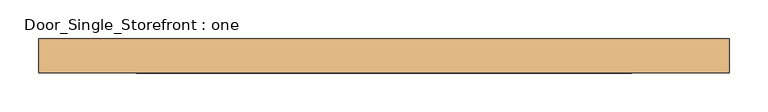
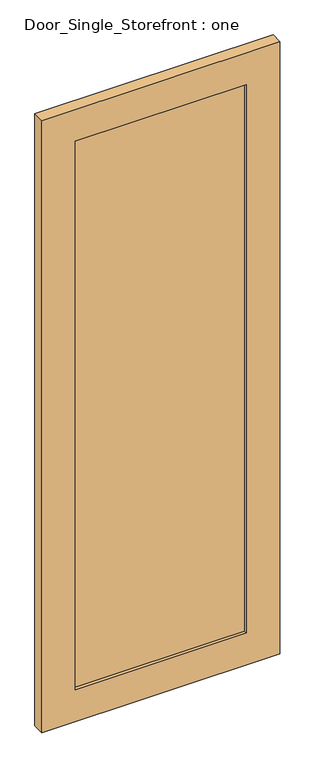
"""IFC4 building model written with IfcOpenShell, lengths in millimetres: door geometry, Door_Single_Storefront : one."""

from ifc_helpers import new_model, si_unit, frame, origin, place, context, project, spatial, polyline, outline, extrude, source, transform, mapped, element, save


def door_single_storefront_one_af52fb56(model_context):
    return source(origin(), model_context, "Body", "SweptSolid", [
        extrude(outline(polyline([(321.46875, -6.35), (-321.46875, -6.35), (-321.46875, 12.7), (321.46875, 12.7), (321.46875, -6.35)])), frame((0.0, 0.0, 127.0), z_axis=(0.0, 0.0, 1.0), x_axis=(1.0, 0.0, 0.0)), (0.0, 0.0, 1.0), 2184.4),
        extrude(outline(polyline([(2438.4, -448.46875), (0.0, -448.46875), (0.0, 448.46875), (2438.4, 448.46875), (2438.4, -448.46875)]), holes=[polyline([(127.0, 321.46875), (127.0, -321.46875), (2311.4, -321.46875), (2311.4, 321.46875), (127.0, 321.46875)])]), frame((0.0, -19.05, 0.0), z_axis=(0.0, 1.0, 0.0), x_axis=(0.0, 0.0, 1.0)), (0.0, 0.0, 1.0), 44.45),
    ])


if __name__ == "__main__":
    model = new_model("IFC4")
    model_context = context("Model", 3, world=origin())
    ifc_project = project(units=[si_unit("LENGTHUNIT", "METRE", prefix="MILLI")], contexts=[model_context])
    site = spatial("IfcSite", under=ifc_project)
    building = spatial("IfcBuilding", under=site)
    placement = place(None, origin())
    door_single_storefront_one_shape = door_single_storefront_one_af52fb56(model_context)
    element("IfcDoor", 1, ObjectType="Door_Single_Storefront : one", at=placement, inside=building, context=model_context, shape_type="MappedRepresentation", body=[
        mapped(door_single_storefront_one_shape, transform((0.0, 0.0, 0.0), x_axis=(1.0, 0.0, 0.0), y_axis=(0.0, 1.0, 0.0), z_axis=(0.0, 0.0, 1.0))),
    ])
    save(model, "model.ifc")

# Revit data of these elements
# Type "Door_Single_Storefront : one"
#   Type Mark = "27"
#   Analytic Construction = "<None>"
#   Stile_Width = 0' - 5"
#   Door_Thickness = 0' - 1 3/4"
#   Door_Offset = 0' - 1"
#   Glass_Material = SAFETY GLAZING
#   Frame_Material = INTERIOR GRADE ALUMINUM STOREFRONT W/ SAFETY GLAZING
#   Function = (empty or 0)
# Element 1 (IfcDoor, "Door_Single_Storefront : one")
#   Materials on its faces: "INTERIOR GRADE ALUMINUM STOREFRONT W/ SAFETY GLAZING", "SAFETY GLAZING"
# Materials
#   "SAFETY GLAZING": class "Glass", colour RGB 142 168 196, transparency 0.75, Description = "Soda Lime Glass", Cost = 0
#   "INTERIOR GRADE ALUMINUM STOREFRONT W/ SAFETY GLAZING": class "Metal", colour RGB 226 226 226, transparency 0, Description = "Aluminum 6061", Cost = 0
